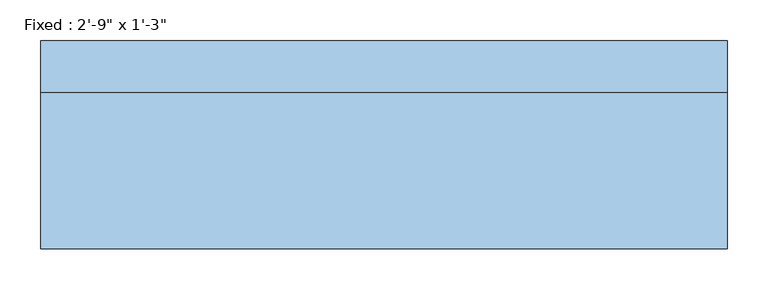
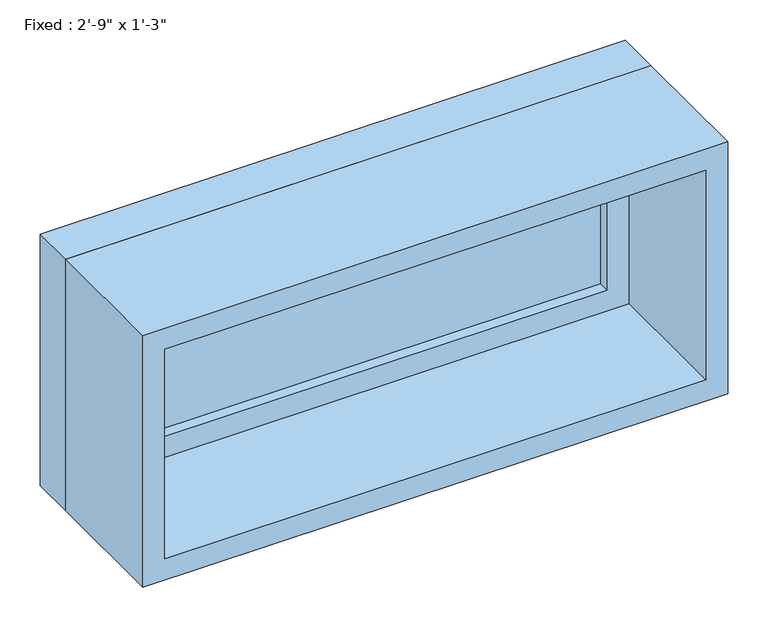
"""IFC4 building model written with IfcOpenShell, lengths in millimetres: window geometry."""

from ifc_helpers import new_model, si_unit, frame, origin, place, context, project, spatial, polyline, outline, extrude, source, transform, mapped, element, save


def window_bf5cd34b(model_context):
    return source(origin(), model_context, "Body", "SweptSolid", [
        extrude(outline(polyline([(317.5, 79.375), (-393.7, 79.375), (-393.7, 92.075), (317.5, 92.075), (317.5, 79.375)])), frame((0.0, 0.0, 977.9), z_axis=(0.0, 0.0, 1.0), x_axis=(1.0, 0.0, 0.0)), (0.0, 0.0, 1.0), 254.0),
        extrude(outline(polyline([(1276.35, -438.15), (933.45, -438.15), (933.45, 361.95), (1276.35, 361.95), (1276.35, -438.15)]), holes=[polyline([(1231.9, -393.7), (1231.9, 317.5), (977.9, 317.5), (977.9, -393.7), (1231.9, -393.7)])]), frame((0.0, 63.5, 0.0), z_axis=(0.0, 1.0, 0.0), x_axis=(0.0, 0.0, 1.0)), (0.0, 0.0, 1.0), 44.45),
        extrude(outline(polyline([(1295.4, -457.2), (914.4, -457.2), (914.4, 381.0), (1295.4, 381.0), (1295.4, -457.2)]), holes=[polyline([(1263.65, -425.45), (1263.65, 349.25), (946.15, 349.25), (946.15, -425.45), (1263.65, -425.45)])]), frame((0.0, -127.0, 0.0), z_axis=(0.0, 1.0, 0.0), x_axis=(0.0, 0.0, 1.0)), (0.0, 0.0, 1.0), 190.5),
        extrude(outline(polyline([(1295.4, 381.0), (1295.4, -457.2), (914.4, -457.2), (914.4, 381.0), (1295.4, 381.0)]), holes=[polyline([(1276.35, 361.95), (933.45, 361.95), (933.45, -438.15), (1276.35, -438.15), (1276.35, 361.95)])]), frame((0.0, 63.5, 0.0), z_axis=(0.0, 1.0, 0.0), x_axis=(0.0, 0.0, 1.0)), (0.0, 0.0, 1.0), 63.5),
    ])


if __name__ == "__main__":
    model = new_model("IFC4")
    model_context = context("Model", 3, world=origin())
    ifc_project = project(units=[si_unit("LENGTHUNIT", "METRE", prefix="MILLI")], contexts=[model_context])
    site = spatial("IfcSite", under=ifc_project)
    building = spatial("IfcBuilding", under=site)
    placement = place(None, origin())
    window_shape = window_bf5cd34b(model_context)
    element("IfcWindow", 1, ObjectType="Fixed : 2'-9\" x 1'-3\"", at=placement, inside=building, context=model_context, shape_type="MappedRepresentation", body=[
        mapped(window_shape, transform((0.0, 0.0, 0.0), x_axis=(1.0, 0.0, 0.0), y_axis=(0.0, 1.0, 0.0), z_axis=(0.0, 0.0, 1.0))),
    ])
    save(model, "model.ifc")

# Revit data of these elements
# Type "Fixed : 2'-9\" x 1'-3\""
#   Type Mark = "29"
#   Construction Type Id = "GSP4R"
#   Assembly Code = "B2020100"
#   Analytic Construction = "1/8 in Pilkington single glazing"
#   Visual Light Transmittance = 0.9
#   Solar Heat Gain Coefficient = 0.78
#   Heat Transfer Coefficient (U) = 3.6886 W/(m²·K)
#   Height = 1' - 3"
#   Default Sill Height = 3' - 0"
#   Width = 2' - 9"
#   Window Inset = 0' - 0 3/4"
#   Glass Pane Material = Glass
#   Sash Material = Sash
#   Wall Closure = (empty or 0)
# Element 1 (IfcWindow, "Fixed : 2'-9\" x 1'-3\"")
#   Materials on its faces: "Sash", "Glass"
# Materials
#   "Glass": class "Glass", colour RGB 0 128 192, transparency 0.75, Description = "Soda Lime Glass", Cost = 0
#   "Sash": class "Wood", colour RGB 224 178 126, transparency 0, Cost = 0
